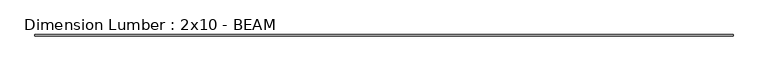
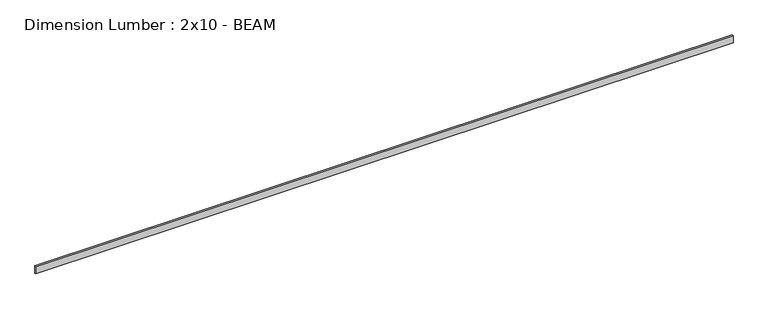
"""IFC4 building model written with IfcOpenShell, lengths in millimetres: beam geometry, Dimension Lumber : 2x10 - BEAM."""

from ifc_helpers import new_model, si_unit, frame, origin, place, context, project, spatial, polyline, outline, extrude, source, transform, mapped, element, save


def dimension_lumber_2x10_beam_cea37807(model_context):
    return source(origin(), model_context, "Body", "SweptSolid", [
        extrude(outline(polyline([(10510.04375, 19.05), (10510.04375, -19.05), (-10619.58125, -19.05), (-10619.58125, 19.05), (10510.04375, 19.05)])), frame((0.0, 0.0, -117.475), z_axis=(0.0, 0.0, 1.0), x_axis=(1.0, 0.0, 0.0)), (0.0, 0.0, 1.0), 234.95),
    ])


if __name__ == "__main__":
    model = new_model("IFC4")
    model_context = context("Model", 3, world=origin())
    ifc_project = project(units=[si_unit("LENGTHUNIT", "METRE", prefix="MILLI")], contexts=[model_context])
    site = spatial("IfcSite", under=ifc_project)
    building = spatial("IfcBuilding", under=site)
    placement = place(None, origin())
    dimension_lumber_2x10_beam_shape = dimension_lumber_2x10_beam_cea37807(model_context)
    element("IfcBeam", 1, ObjectType="Dimension Lumber : 2x10 - BEAM", at=placement, inside=building, context=model_context, shape_type="MappedRepresentation", body=[
        mapped(dimension_lumber_2x10_beam_shape, transform((0.0, 0.0, 0.0), x_axis=(1.0, 0.0, 0.0), y_axis=(0.0, 1.0, 0.0), z_axis=(0.0, 0.0, 1.0))),
    ])
    save(model, "model.ifc")

# Revit data of these elements
# Type "Dimension Lumber : 2x10 - BEAM"
#   Assembly Code = "B10"
#   A = 0.0755556 SF
#   Length [instance default] = 5' - 0"
#   b = 0' - 1 1/2"
#   d = 0' - 9 1/4"
#   Structural Material = (3) SISTERED 2X10s AT BEAM
# Element 1 (IfcBeam, "Dimension Lumber : 2x10 - BEAM")
#   Materials on its faces: "(3) SISTERED 2X10s AT BEAM"
# Materials
#   "(3) SISTERED 2X10s AT BEAM": class "Wood", colour RGB 234 198 147, transparency 0, Description = "Pinus Echinata", Cost = 0
